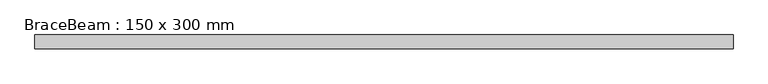
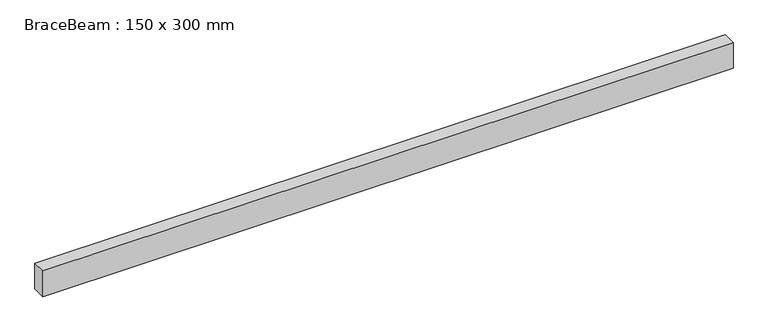
"""IFC4 building model written with IfcOpenShell, lengths in millimetres: beam geometry, BraceBeam : 150 x 300 mm."""

from ifc_helpers import new_model, si_unit, frame, origin, place, context, project, spatial, polyline, outline, extrude, source, transform, mapped, element, save


def bracebeam_150_x_300_mm_571b2135(model_context):
    return source(origin(), model_context, "Body", "SweptSolid", [
        extrude(outline(polyline([(-3800.0, -75.0), (-3800.0, 75.0), (3800.0, 75.0), (3800.0, -75.0), (-3800.0, -75.0)])), frame((0.0, 0.0, -150.0), z_axis=(0.0, 0.0, 1.0), x_axis=(1.0, 0.0, 0.0)), (0.0, 0.0, 1.0), 300.0),
    ])


if __name__ == "__main__":
    model = new_model("IFC4")
    model_context = context("Model", 3, world=origin())
    ifc_project = project(units=[si_unit("LENGTHUNIT", "METRE", prefix="MILLI")], contexts=[model_context])
    site = spatial("IfcSite", under=ifc_project)
    building = spatial("IfcBuilding", under=site)
    placement = place(None, origin())
    bracebeam_150_x_300_mm_shape = bracebeam_150_x_300_mm_571b2135(model_context)
    element("IfcBeam", 1, ObjectType="BraceBeam : 150 x 300 mm", at=placement, inside=building, context=model_context, shape_type="MappedRepresentation", body=[
        mapped(bracebeam_150_x_300_mm_shape, transform((0.0, 0.0, 0.0), x_axis=(1.0, 0.0, 0.0), y_axis=(0.0, 1.0, 0.0), z_axis=(0.0, 0.0, 1.0))),
    ])
    save(model, "model.ifc")

# Revit data of these elements
# Type "BraceBeam : 150 x 300 mm"
#   ExpertTruss = "Height\th\r\nWidth\tb"
#   Name [instance default] = ""
#   m [instance default] = 0 mm
#   ip_c_cut_control [instance default] = 1300 mm
#   ip_c_cut [instance default] = 1300 mm
#   h_fix [instance default] = 900 mm
#   d/2 [instance default] = 1750 mm
#   c_cut_incl [instance default] = -1000 mm
#   c_cut [instance default] = 0 mm
#   beta0_2 [instance default] = 90.00°
#   beta0_1 [instance default] = 90.00°
#   alfaMax [instance default] = 0.00°
#   alfa0_2 [instance default] = 90.00°
#   ZOffsetStr_0 [instance default] = 150 mm
#   ZOffsetStr [instance default] = 0 mm
#   ZOffsetEnd_0 [instance default] = 150 mm
#   ZOffsetEnd [instance default] = 0 mm
#   Beta2 [instance default] = 0.00°
#   Beta1 [instance default] = 0.00°
#   Alfa_str [instance default] = 0.00°
#   Alfa_cut_control [instance default] = 90.00°
#   Alfa_cut [instance default] = 90.00°
#   AlfaMAX [instance default] = 0.00°
#   Alfa2_0 [instance default] = 0.00°
#   Alfa2 [instance default] = 0.00°
#   Alfa1_0 [instance default] = 0.00°
#   Alfa1 [instance default] = 0.00°
#   A_max_Str [instance default] = 0.00°
#   h_void [instance default] = 3000 mm
#   beam_L_0 [instance default] = 100 mm
#   beam_L [instance default] = 0 mm
#   b_void [instance default] = 160 mm
#   alfa0_1 [instance default] = 90.00°
#   b = 150 mm
#   YOffsetStr [instance default] = 0 mm
#   YOffsetEnd [instance default] = 0 mm
#   XOffsetStr_0 [instance default] = 3500 mm
#   XOffsetStr [instance default] = 0 mm
#   XOffsetEnd_0 [instance default] = 3500 mm
#   XOffsetEnd [instance default] = 0 mm
#   L_void_0 [instance default] = 100 mm
#   L_void [instance default] = 0 mm
#   E2 [instance default] = 0.00°
#   E1 [instance default] = 0.00°
#   Length [instance default] = 3500 mm
#   h = 300 mm
#   Alfa [instance default] = 0.00°
#   A_max_End [instance default] = 0.00°
#   A_max [instance default] = 0.00°
#   A4 [instance default] = 0.00°
#   A3 [instance default] = 0.00°
#   A2 [instance default] = 0.00°
#   A1 [instance default] = 0.00°
#   BetaAngles [instance default] = no
#   Material [instance default] = Wood Standard
# Element 1 (IfcBeam, "BraceBeam : 150 x 300 mm")
#   d/2 = 3650 mm
#   XOffsetStr_0 = 7450 mm
#   XOffsetStr = -150 mm
#   XOffsetEnd_0 = 7450 mm
#   XOffsetEnd = -150 mm
#   Materials on its faces: "Wood Standard"
# Materials
#   "Wood Standard": class "Drewno", colour RGB 196 146 67, transparency 0, Cost = 0
